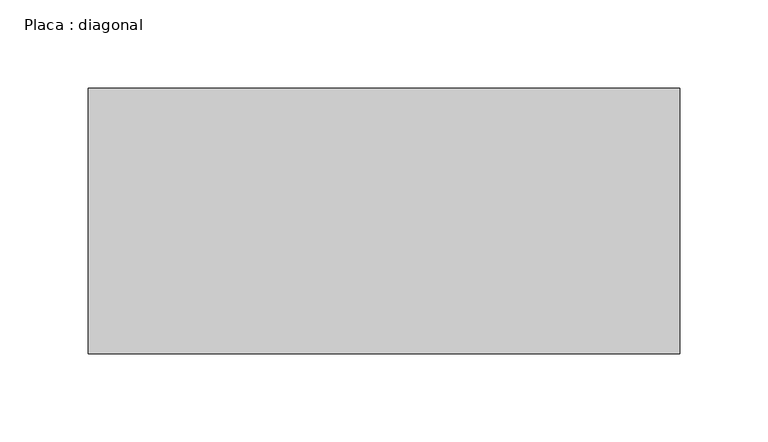
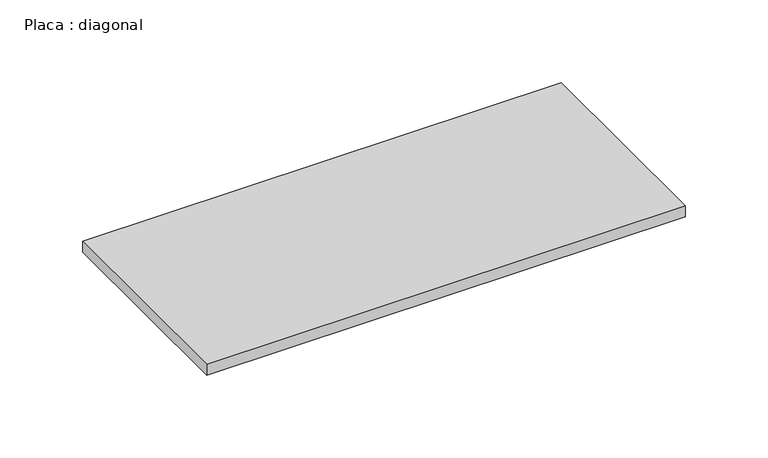
"""IFC4 building model written with IfcOpenShell, lengths in millimetres: beam geometry, Placa : diagonal."""

from ifc_helpers import new_model, si_unit, frame, origin, place, context, project, spatial, polyline, outline, extrude, source, transform, mapped, element, save


def placa_diagonal_4478edde(model_context):
    return source(origin(), model_context, "Body", "SweptSolid", [
        extrude(outline(polyline([(167.0675392, 75.0), (167.0675392, -75.0), (-167.4240165, -75.0), (-167.4240165, 75.0), (167.0675392, 75.0)])), frame((0.0, 0.0, -4.0), z_axis=(0.0, 0.0, 1.0), x_axis=(1.0, 0.0, 0.0)), (0.0, 0.0, 1.0), 8.0),
    ])


if __name__ == "__main__":
    model = new_model("IFC4")
    model_context = context("Model", 3, world=origin())
    ifc_project = project(units=[si_unit("LENGTHUNIT", "METRE", prefix="MILLI")], contexts=[model_context])
    site = spatial("IfcSite", under=ifc_project)
    building = spatial("IfcBuilding", under=site)
    placement = place(None, origin())
    placa_diagonal_shape = placa_diagonal_4478edde(model_context)
    element("IfcBeam", 1, ObjectType="Placa : diagonal", at=placement, inside=building, context=model_context, shape_type="MappedRepresentation", body=[
        mapped(placa_diagonal_shape, transform((0.0, 0.0, 0.0), x_axis=(1.0, 0.0, 0.0), y_axis=(0.0, 1.0, 0.0), z_axis=(0.0, 0.0, 1.0))),
    ])
    save(model, "model.ifc")

# Revit data of these elements
# Type "Placa : diagonal"
#   W = 0
#   Length [instance default] = 1.50 m
#   b = 0.15 m
#   d = 0.008 m
#   A = 0 m²
#   Structural Material [instance default] = Aço, 45-345
# Element 1 (IfcBeam, "Placa : diagonal")
#   Materials on its faces: "Aço, 45-345"
# Materials
#   "Aço, 45-345": class "Metal", colour RGB 247 247 247, transparency 0, Description = "Aço 345 MPa", Cost = 0
